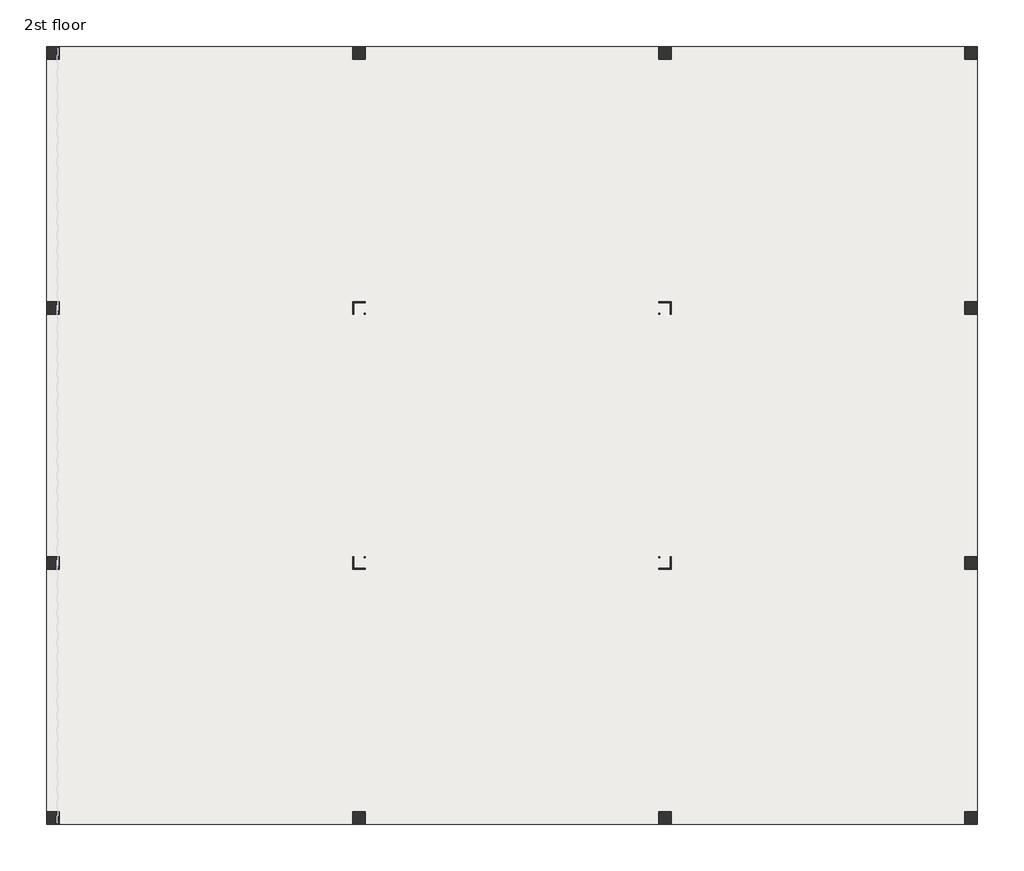
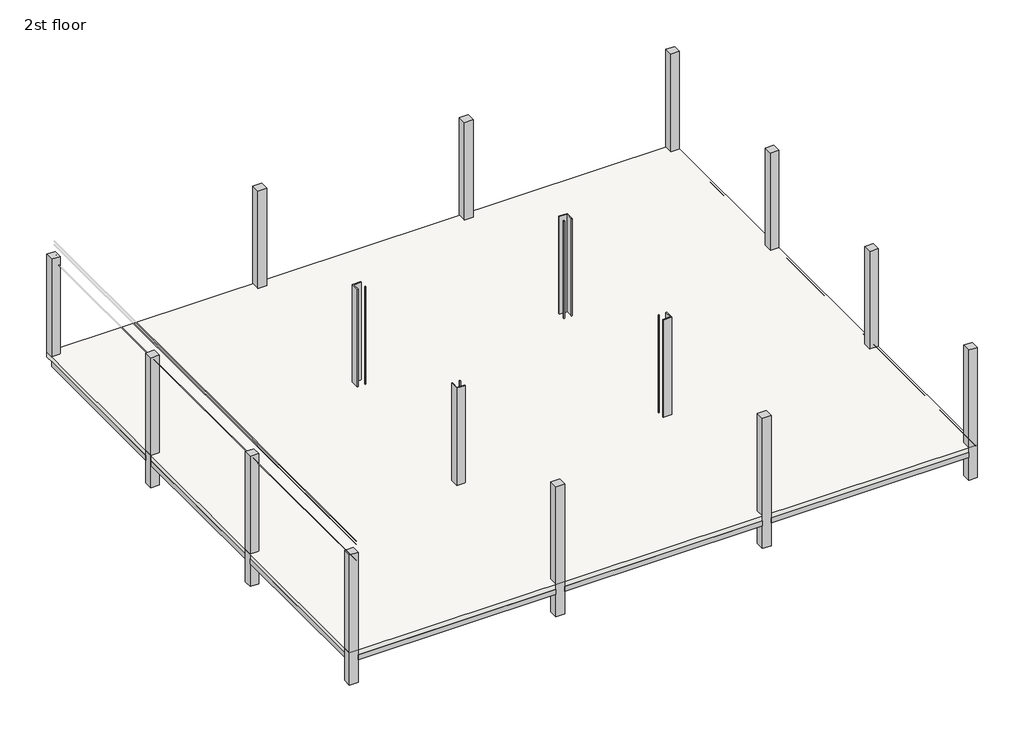
# One storey, part 1 of 2: 24 beams, 16 columns, 1 slab.
"""IFC4 building model written with IfcOpenShell, lengths in millimetres."""

from ifc_helpers import new_model, si_unit, frame, origin, place, context, project, spatial, polyline, outline, extrude, faceted_brep, element, save

model = new_model("IFC4")

# Units and contexts
model_context = context("Model", 3, world=origin())
ifc_project = project(units=[si_unit("LENGTHUNIT", "METRE", prefix="MILLI")], contexts=[model_context])

# Site, building, storey
site = spatial("IfcSite", under=ifc_project)
building = spatial("IfcBuilding", under=site)
storey = spatial("IfcBuildingStorey", under=building, Name="2st floor", Elevation=8500.0)

# Beams
placement = place(None, origin())
element("IfcBeam", 1, ObjectType="Concrete-Rectangular Beam : 250 x 300mm", at=placement, inside=storey, context=model_context, shape_type="SweptSolid", body=[
    extrude(outline(polyline([(-3083.7181639, -5443.2383613), (-3083.7181639, -5693.2383613), (-8833.7181639, -5693.2383613), (-8833.7181639, -5443.2383613), (-3083.7181639, -5443.2383613)])), frame((0.0, 0.0, 8200.0), z_axis=(0.0, 0.0, 1.0), x_axis=(1.0, 0.0, 0.0)), (0.0, 0.0, 1.0), 150.0),
])
element("IfcBeam", 2, ObjectType="Concrete-Rectangular Beam : 250 x 300mm", at=placement, inside=storey, context=model_context, shape_type="SweptSolid", body=[
    extrude(outline(polyline([(-2833.7181639, -5693.2383613), (-2833.7181639, -5443.2383613), (2916.2818361, -5443.2383613), (2916.2818361, -5693.2383613), (-2833.7181639, -5693.2383613)])), frame((0.0, 0.0, 8200.0), z_axis=(0.0, 0.0, 1.0), x_axis=(1.0, 0.0, 0.0)), (0.0, 0.0, 1.0), 150.0),
])
element("IfcBeam", 3, ObjectType="Concrete-Rectangular Beam : 250 x 300mm", at=placement, inside=storey, context=model_context, shape_type="SweptSolid", body=[
    extrude(outline(polyline([(3166.2818361, -5693.2383613), (3166.2818361, -5443.2383613), (8916.2818361, -5443.2383613), (8916.2818361, -5693.2383613), (3166.2818361, -5693.2383613)])), frame((0.0, 0.0, 8200.0), z_axis=(0.0, 0.0, 1.0), x_axis=(1.0, 0.0, 0.0)), (0.0, 0.0, 1.0), 150.0),
])
element("IfcBeam", 4, ObjectType="Concrete-Rectangular Beam : 250 x 300mm", at=placement, inside=storey, context=model_context, shape_type="SweptSolid", body=[
    extrude(outline(polyline([(-8833.7181639, -10443.2383613), (-9083.7181639, -10443.2383613), (-9083.7181639, -5693.2383613), (-8833.7181639, -5693.2383613), (-8833.7181639, -10443.2383613)])), frame((0.0, 0.0, 8200.0), z_axis=(0.0, 0.0, 1.0), x_axis=(1.0, 0.0, 0.0)), (0.0, 0.0, 1.0), 150.0),
])
element("IfcBeam", 5, ObjectType="Concrete-Rectangular Beam : 250 x 300mm", at=placement, inside=storey, context=model_context, shape_type="SweptSolid", body=[
    extrude(outline(polyline([(-8833.7181639, -15443.2383613), (-9083.7181639, -15443.2383613), (-9083.7181639, -10693.2383613), (-8833.7181639, -10693.2383613), (-8833.7181639, -15443.2383613)])), frame((0.0, 0.0, 8200.0), z_axis=(0.0, 0.0, 1.0), x_axis=(1.0, 0.0, 0.0)), (0.0, 0.0, 1.0), 150.0),
])
element("IfcBeam", 6, ObjectType="Concrete-Rectangular Beam : 250 x 300mm", at=placement, inside=storey, context=model_context, shape_type="SweptSolid", body=[
    extrude(outline(polyline([(-8833.7181639, -20443.2383613), (-9083.7181639, -20443.2383613), (-9083.7181639, -15693.2383613), (-8833.7181639, -15693.2383613), (-8833.7181639, -20443.2383613)])), frame((0.0, 0.0, 8200.0), z_axis=(0.0, 0.0, 1.0), x_axis=(1.0, 0.0, 0.0)), (0.0, 0.0, 1.0), 150.0),
])
element("IfcBeam", 7, ObjectType="Concrete-Rectangular Beam : 250 x 300mm", at=placement, inside=storey, context=model_context, shape_type="SweptSolid", body=[
    extrude(outline(polyline([(-2833.7181639, -10443.2383613), (-3083.7181639, -10443.2383613), (-3083.7181639, -5693.2383613), (-2833.7181639, -5693.2383613), (-2833.7181639, -10443.2383613)])), frame((0.0, 0.0, 8200.0), z_axis=(0.0, 0.0, 1.0), x_axis=(1.0, 0.0, 0.0)), (0.0, 0.0, 1.0), 150.0),
])
element("IfcBeam", 8, ObjectType="Concrete-Rectangular Beam : 250 x 300mm", at=placement, inside=storey, context=model_context, shape_type="SweptSolid", body=[
    extrude(outline(polyline([(-3083.7181639, -15443.2383613), (-3083.7181639, -10693.2383613), (-3058.7181639, -10693.2383613), (-3058.7181639, -15443.2383613), (-3083.7181639, -15443.2383613)])), frame((0.0, 0.0, 8200.0), z_axis=(0.0, 0.0, 1.0), x_axis=(1.0, 0.0, 0.0)), (0.0, 0.0, 1.0), 150.0),
    extrude(outline(polyline([(-2833.7181639, -10693.2383613), (-2833.7181639, -15443.2383613), (-2858.7181639, -15443.2383613), (-2858.7181639, -10693.2383613), (-2833.7181639, -10693.2383613)])), frame((0.0, 0.0, 8200.0), z_axis=(0.0, 0.0, 1.0), x_axis=(1.0, 0.0, 0.0)), (0.0, 0.0, 1.0), 150.0),
])
element("IfcBeam", 9, ObjectType="Concrete-Rectangular Beam : 250 x 300mm", at=placement, inside=storey, context=model_context, shape_type="SweptSolid", body=[
    extrude(outline(polyline([(-2833.7181639, -20443.2383613), (-3083.7181639, -20443.2383613), (-3083.7181639, -15693.2383613), (-2833.7181639, -15693.2383613), (-2833.7181639, -20443.2383613)])), frame((0.0, 0.0, 8200.0), z_axis=(0.0, 0.0, 1.0), x_axis=(1.0, 0.0, 0.0)), (0.0, 0.0, 1.0), 150.0),
])
element("IfcBeam", 10, ObjectType="Concrete-Rectangular Beam : 250 x 300mm", at=placement, inside=storey, context=model_context, shape_type="SweptSolid", body=[
    extrude(outline(polyline([(3166.2818361, -10443.2383613), (2916.2818361, -10443.2383613), (2916.2818361, -5693.2383613), (3166.2818361, -5693.2383613), (3166.2818361, -10443.2383613)])), frame((0.0, 0.0, 8200.0), z_axis=(0.0, 0.0, 1.0), x_axis=(1.0, 0.0, 0.0)), (0.0, 0.0, 1.0), 150.0),
])
element("IfcBeam", 11, ObjectType="Concrete-Rectangular Beam : 250 x 300mm", at=placement, inside=storey, context=model_context, shape_type="SweptSolid", body=[
    extrude(outline(polyline([(2916.2818361, -15443.2383613), (2916.2818361, -10693.2383613), (2941.2818361, -10693.2383613), (2941.2818361, -15443.2383613), (2916.2818361, -15443.2383613)])), frame((0.0, 0.0, 8200.0), z_axis=(0.0, 0.0, 1.0), x_axis=(1.0, 0.0, 0.0)), (0.0, 0.0, 1.0), 150.0),
    extrude(outline(polyline([(3166.2818361, -10693.2383613), (3166.2818361, -15443.2383613), (3141.2818361, -15443.2383613), (3141.2818361, -10693.2383613), (3166.2818361, -10693.2383613)])), frame((0.0, 0.0, 8200.0), z_axis=(0.0, 0.0, 1.0), x_axis=(1.0, 0.0, 0.0)), (0.0, 0.0, 1.0), 150.0),
])
element("IfcBeam", 12, ObjectType="Concrete-Rectangular Beam : 250 x 300mm", at=placement, inside=storey, context=model_context, shape_type="SweptSolid", body=[
    extrude(outline(polyline([(3166.2818361, -20443.2383613), (2916.2818361, -20443.2383613), (2916.2818361, -15693.2383613), (3166.2818361, -15693.2383613), (3166.2818361, -20443.2383613)])), frame((0.0, 0.0, 8200.0), z_axis=(0.0, 0.0, 1.0), x_axis=(1.0, 0.0, 0.0)), (0.0, 0.0, 1.0), 150.0),
])
element("IfcBeam", 13, ObjectType="Concrete-Rectangular Beam : 250 x 300mm", at=placement, inside=storey, context=model_context, shape_type="SweptSolid", body=[
    extrude(outline(polyline([(9166.2818361, -10443.2383613), (8916.2818361, -10443.2383613), (8916.2818361, -5693.2383613), (9166.2818361, -5693.2383613), (9166.2818361, -10443.2383613)])), frame((0.0, 0.0, 8200.0), z_axis=(0.0, 0.0, 1.0), x_axis=(1.0, 0.0, 0.0)), (0.0, 0.0, 1.0), 150.0),
])
element("IfcBeam", 14, ObjectType="Concrete-Rectangular Beam : 250 x 300mm", at=placement, inside=storey, context=model_context, shape_type="SweptSolid", body=[
    extrude(outline(polyline([(9166.2818361, -15443.2383613), (8916.2818361, -15443.2383613), (8916.2818361, -10693.2383613), (9166.2818361, -10693.2383613), (9166.2818361, -15443.2383613)])), frame((0.0, 0.0, 8200.0), z_axis=(0.0, 0.0, 1.0), x_axis=(1.0, 0.0, 0.0)), (0.0, 0.0, 1.0), 150.0),
])
element("IfcBeam", 15, ObjectType="Concrete-Rectangular Beam : 250 x 300mm", at=placement, inside=storey, context=model_context, shape_type="SweptSolid", body=[
    extrude(outline(polyline([(9166.2818361, -20443.2383613), (8916.2818361, -20443.2383613), (8916.2818361, -15693.2383613), (9166.2818361, -15693.2383613), (9166.2818361, -20443.2383613)])), frame((0.0, 0.0, 8200.0), z_axis=(0.0, 0.0, 1.0), x_axis=(1.0, 0.0, 0.0)), (0.0, 0.0, 1.0), 150.0),
])
element("IfcBeam", 16, ObjectType="Concrete-Rectangular Beam : 250 x 300mm", at=placement, inside=storey, context=model_context, shape_type="SweptSolid", body=[
    extrude(outline(polyline([(-8833.7181639, -20693.2383613), (-8833.7181639, -20443.2383613), (-3083.7181639, -20443.2383613), (-3083.7181639, -20693.2383613), (-8833.7181639, -20693.2383613)])), frame((0.0, 0.0, 8200.0), z_axis=(0.0, 0.0, 1.0), x_axis=(1.0, 0.0, 0.0)), (0.0, 0.0, 1.0), 150.0),
])
element("IfcBeam", 17, ObjectType="Concrete-Rectangular Beam : 250 x 300mm", at=placement, inside=storey, context=model_context, shape_type="SweptSolid", body=[
    extrude(outline(polyline([(-2833.7181639, -20693.2383613), (-2833.7181639, -20443.2383613), (2916.2818361, -20443.2383613), (2916.2818361, -20693.2383613), (-2833.7181639, -20693.2383613)])), frame((0.0, 0.0, 8200.0), z_axis=(0.0, 0.0, 1.0), x_axis=(1.0, 0.0, 0.0)), (0.0, 0.0, 1.0), 150.0),
])
element("IfcBeam", 18, ObjectType="Concrete-Rectangular Beam : 250 x 300mm", at=placement, inside=storey, context=model_context, shape_type="SweptSolid", body=[
    extrude(outline(polyline([(3166.2818361, -20693.2383613), (3166.2818361, -20443.2383613), (8916.2818361, -20443.2383613), (8916.2818361, -20693.2383613), (3166.2818361, -20693.2383613)])), frame((0.0, 0.0, 8200.0), z_axis=(0.0, 0.0, 1.0), x_axis=(1.0, 0.0, 0.0)), (0.0, 0.0, 1.0), 150.0),
])
element("IfcBeam", 19, ObjectType="Concrete-Rectangular Beam : 250 x 300mm", at=placement, inside=storey, context=model_context, shape_type="SweptSolid", body=[
    extrude(outline(polyline([(-8833.7181639, -15693.2383613), (-8833.7181639, -15443.2383613), (-3083.7181639, -15443.2383613), (-3083.7181639, -15693.2383613), (-8833.7181639, -15693.2383613)])), frame((0.0, 0.0, 8200.0), z_axis=(0.0, 0.0, 1.0), x_axis=(1.0, 0.0, 0.0)), (0.0, 0.0, 1.0), 150.0),
])
element("IfcBeam", 20, ObjectType="Concrete-Rectangular Beam : 250 x 300mm", at=placement, inside=storey, context=model_context, shape_type="SweptSolid", body=[
    extrude(outline(polyline([(2916.2818361, -15693.2383613), (-2833.7181639, -15693.2383613), (-2833.7181639, -15668.2383613), (2916.2818361, -15668.2383613), (2916.2818361, -15693.2383613)])), frame((0.0, 0.0, 8200.0), z_axis=(0.0, 0.0, 1.0), x_axis=(1.0, 0.0, 0.0)), (0.0, 0.0, 1.0), 150.0),
    extrude(outline(polyline([(-2833.7181639, -15443.2383613), (2916.2818361, -15443.2383613), (2916.2818361, -15468.2383613), (-2833.7181639, -15468.2383613), (-2833.7181639, -15443.2383613)])), frame((0.0, 0.0, 8200.0), z_axis=(0.0, 0.0, 1.0), x_axis=(1.0, 0.0, 0.0)), (0.0, 0.0, 1.0), 150.0),
])
element("IfcBeam", 21, ObjectType="Concrete-Rectangular Beam : 250 x 300mm", at=placement, inside=storey, context=model_context, shape_type="SweptSolid", body=[
    extrude(outline(polyline([(3166.2818361, -15693.2383613), (3166.2818361, -15443.2383613), (8916.2818361, -15443.2383613), (8916.2818361, -15693.2383613), (3166.2818361, -15693.2383613)])), frame((0.0, 0.0, 8200.0), z_axis=(0.0, 0.0, 1.0), x_axis=(1.0, 0.0, 0.0)), (0.0, 0.0, 1.0), 150.0),
])
element("IfcBeam", 22, ObjectType="Concrete-Rectangular Beam : 250 x 300mm", at=placement, inside=storey, context=model_context, shape_type="SweptSolid", body=[
    extrude(outline(polyline([(-8833.7181639, -10693.2383613), (-8833.7181639, -10443.2383613), (-3083.7181639, -10443.2383613), (-3083.7181639, -10693.2383613), (-8833.7181639, -10693.2383613)])), frame((0.0, 0.0, 8200.0), z_axis=(0.0, 0.0, 1.0), x_axis=(1.0, 0.0, 0.0)), (0.0, 0.0, 1.0), 150.0),
])
element("IfcBeam", 23, ObjectType="Concrete-Rectangular Beam : 250 x 300mm", at=placement, inside=storey, context=model_context, shape_type="SweptSolid", body=[
    extrude(outline(polyline([(2916.2818361, -10693.2383613), (-2833.7181639, -10693.2383613), (-2833.7181639, -10668.2383613), (2916.2818361, -10668.2383613), (2916.2818361, -10693.2383613)])), frame((0.0, 0.0, 8200.0), z_axis=(0.0, 0.0, 1.0), x_axis=(1.0, 0.0, 0.0)), (0.0, 0.0, 1.0), 150.0),
    extrude(outline(polyline([(-2833.7181639, -10443.2383613), (2916.2818361, -10443.2383613), (2916.2818361, -10468.2383613), (-2833.7181639, -10468.2383613), (-2833.7181639, -10443.2383613)])), frame((0.0, 0.0, 8200.0), z_axis=(0.0, 0.0, 1.0), x_axis=(1.0, 0.0, 0.0)), (0.0, 0.0, 1.0), 150.0),
])
element("IfcBeam", 24, ObjectType="Concrete-Rectangular Beam : 250 x 300mm", at=placement, inside=storey, context=model_context, shape_type="SweptSolid", body=[
    extrude(outline(polyline([(3166.2818361, -10693.2383613), (3166.2818361, -10443.2383613), (8916.2818361, -10443.2383613), (8916.2818361, -10693.2383613), (3166.2818361, -10693.2383613)])), frame((0.0, 0.0, 8200.0), z_axis=(0.0, 0.0, 1.0), x_axis=(1.0, 0.0, 0.0)), (0.0, 0.0, 1.0), 150.0),
])

# Columns
element("IfcColumn", 25, ObjectType="Concrete-Rectangular-Column : 250x250 mm", at=placement, inside=storey, context=model_context, shape_type="SweptSolid", body=[
    extrude(outline(polyline([(-8833.7181639, -20443.2383613), (-8833.7181639, -20693.2383613), (-9083.7181639, -20693.2383613), (-9083.7181639, -20443.2383613), (-8833.7181639, -20443.2383613)])), frame((0.0, 0.0, 7500.0), z_axis=(0.0, 0.0, 1.0), x_axis=(1.0, 0.0, 0.0)), (0.0, 0.0, 1.0), 4000.0),
])
element("IfcColumn", 26, ObjectType="Concrete-Rectangular-Column : 250x250 mm", at=placement, inside=storey, context=model_context, shape_type="SweptSolid", body=[
    extrude(outline(polyline([(-8833.7181639, -15443.2383613), (-8833.7181639, -15693.2383613), (-9083.7181639, -15693.2383613), (-9083.7181639, -15443.2383613), (-8833.7181639, -15443.2383613)])), frame((0.0, 0.0, 7500.0), z_axis=(0.0, 0.0, 1.0), x_axis=(1.0, 0.0, 0.0)), (0.0, 0.0, 1.0), 4000.0),
])
element("IfcColumn", 27, ObjectType="Concrete-Rectangular-Column : 250x250 mm", at=placement, inside=storey, context=model_context, shape_type="SweptSolid", body=[
    extrude(outline(polyline([(-8833.7181639, -10443.2383613), (-8833.7181639, -10693.2383613), (-9083.7181639, -10693.2383613), (-9083.7181639, -10443.2383613), (-8833.7181639, -10443.2383613)])), frame((0.0, 0.0, 7500.0), z_axis=(0.0, 0.0, 1.0), x_axis=(1.0, 0.0, 0.0)), (0.0, 0.0, 1.0), 4000.0),
])
element("IfcColumn", 28, ObjectType="Concrete-Rectangular-Column : 250x250 mm", at=placement, inside=storey, context=model_context, shape_type="SweptSolid", body=[
    extrude(outline(polyline([(-8833.7181639, -5443.2383613), (-8833.7181639, -5693.2383613), (-9083.7181639, -5693.2383613), (-9083.7181639, -5443.2383613), (-8833.7181639, -5443.2383613)])), frame((0.0, 0.0, 8500.0), z_axis=(0.0, 0.0, 1.0), x_axis=(1.0, 0.0, 0.0)), (0.0, 0.0, 1.0), 3000.0),
])
element("IfcColumn", 29, ObjectType="Concrete-Rectangular-Column : 250x250 mm", at=placement, inside=storey, context=model_context, shape_type="SweptSolid", body=[
    extrude(outline(polyline([(-2833.7181639, -20443.2383613), (-2833.7181639, -20693.2383613), (-3083.7181639, -20693.2383613), (-3083.7181639, -20443.2383613), (-2833.7181639, -20443.2383613)])), frame((0.0, 0.0, 7500.0), z_axis=(0.0, 0.0, 1.0), x_axis=(1.0, 0.0, 0.0)), (0.0, 0.0, 1.0), 4000.0),
])
element("IfcColumn", 30, ObjectType="Concrete-Rectangular-Column : 250x250 mm", at=placement, inside=storey, context=model_context, shape_type="SweptSolid", body=[
    extrude(outline(polyline([(-2833.7181639, -15443.2383613), (-2833.7181639, -15468.2383613), (-2858.7181639, -15468.2383613), (-2858.7181639, -15443.2383613), (-2833.7181639, -15443.2383613)])), frame((0.0, 0.0, 7500.0), z_axis=(0.0, 0.0, 1.0), x_axis=(1.0, 0.0, 0.0)), (0.0, 0.0, 1.0), 4000.0),
    extrude(outline(polyline([(-2833.7181639, -15693.2383613), (-3083.7181639, -15693.2383613), (-3083.7181639, -15443.2383613), (-3058.7181639, -15443.2383613), (-3058.7181639, -15668.2383613), (-2833.7181639, -15668.2383613), (-2833.7181639, -15693.2383613)])), frame((0.0, 0.0, 7500.0), z_axis=(0.0, 0.0, 1.0), x_axis=(1.0, 0.0, 0.0)), (0.0, 0.0, 1.0), 4000.0),
])
element("IfcColumn", 31, ObjectType="Concrete-Rectangular-Column : 250x250 mm", at=placement, inside=storey, context=model_context, shape_type="SweptSolid", body=[
    extrude(outline(polyline([(-3083.7181639, -10693.2383613), (-3083.7181639, -10443.2383613), (-2833.7181639, -10443.2383613), (-2833.7181639, -10468.2383613), (-3058.7181639, -10468.2383613), (-3058.7181639, -10693.2383613), (-3083.7181639, -10693.2383613)])), frame((0.0, 0.0, 7500.0), z_axis=(0.0, 0.0, 1.0), x_axis=(1.0, 0.0, 0.0)), (0.0, 0.0, 1.0), 4000.0),
    extrude(outline(polyline([(-2833.7181639, -10668.2383613), (-2833.7181639, -10693.2383613), (-2858.7181639, -10693.2383613), (-2858.7181639, -10668.2383613), (-2833.7181639, -10668.2383613)])), frame((0.0, 0.0, 7500.0), z_axis=(0.0, 0.0, 1.0), x_axis=(1.0, 0.0, 0.0)), (0.0, 0.0, 1.0), 4000.0),
])
element("IfcColumn", 32, ObjectType="Concrete-Rectangular-Column : 250x250 mm", at=placement, inside=storey, context=model_context, shape_type="SweptSolid", body=[
    extrude(outline(polyline([(-2833.7181639, -5443.2383613), (-2833.7181639, -5693.2383613), (-3083.7181639, -5693.2383613), (-3083.7181639, -5443.2383613), (-2833.7181639, -5443.2383613)])), frame((0.0, 0.0, 7500.0), z_axis=(0.0, 0.0, 1.0), x_axis=(1.0, 0.0, 0.0)), (0.0, 0.0, 1.0), 4000.0),
])
element("IfcColumn", 33, ObjectType="Concrete-Rectangular-Column : 250x250 mm", at=placement, inside=storey, context=model_context, shape_type="SweptSolid", body=[
    extrude(outline(polyline([(3166.2818361, -20443.2383613), (3166.2818361, -20693.2383613), (2916.2818361, -20693.2383613), (2916.2818361, -20443.2383613), (3166.2818361, -20443.2383613)])), frame((0.0, 0.0, 7500.0), z_axis=(0.0, 0.0, 1.0), x_axis=(1.0, 0.0, 0.0)), (0.0, 0.0, 1.0), 4000.0),
])
element("IfcColumn", 34, ObjectType="Concrete-Rectangular-Column : 250x250 mm", at=placement, inside=storey, context=model_context, shape_type="SweptSolid", body=[
    extrude(outline(polyline([(2916.2818361, -15468.2383613), (2916.2818361, -15443.2383613), (2941.2818361, -15443.2383613), (2941.2818361, -15468.2383613), (2916.2818361, -15468.2383613)])), frame((0.0, 0.0, 7500.0), z_axis=(0.0, 0.0, 1.0), x_axis=(1.0, 0.0, 0.0)), (0.0, 0.0, 1.0), 4000.0),
    extrude(outline(polyline([(3166.2818361, -15443.2383613), (3166.2818361, -15693.2383613), (2916.2818361, -15693.2383613), (2916.2818361, -15668.2383613), (3141.2818361, -15668.2383613), (3141.2818361, -15443.2383613), (3166.2818361, -15443.2383613)])), frame((0.0, 0.0, 7500.0), z_axis=(0.0, 0.0, 1.0), x_axis=(1.0, 0.0, 0.0)), (0.0, 0.0, 1.0), 4000.0),
])
element("IfcColumn", 35, ObjectType="Concrete-Rectangular-Column : 250x250 mm", at=placement, inside=storey, context=model_context, shape_type="SweptSolid", body=[
    extrude(outline(polyline([(3166.2818361, -10443.2383613), (3166.2818361, -10693.2383613), (3141.2818361, -10693.2383613), (3141.2818361, -10468.2383613), (2916.2818361, -10468.2383613), (2916.2818361, -10443.2383613), (3166.2818361, -10443.2383613)])), frame((0.0, 0.0, 7500.0), z_axis=(0.0, 0.0, 1.0), x_axis=(1.0, 0.0, 0.0)), (0.0, 0.0, 1.0), 4000.0),
    extrude(outline(polyline([(2916.2818361, -10693.2383613), (2916.2818361, -10668.2383613), (2941.2818361, -10668.2383613), (2941.2818361, -10693.2383613), (2916.2818361, -10693.2383613)])), frame((0.0, 0.0, 7500.0), z_axis=(0.0, 0.0, 1.0), x_axis=(1.0, 0.0, 0.0)), (0.0, 0.0, 1.0), 4000.0),
])
element("IfcColumn", 36, ObjectType="Concrete-Rectangular-Column : 250x250 mm", at=placement, inside=storey, context=model_context, shape_type="SweptSolid", body=[
    extrude(outline(polyline([(3166.2818361, -5443.2383613), (3166.2818361, -5693.2383613), (2916.2818361, -5693.2383613), (2916.2818361, -5443.2383613), (3166.2818361, -5443.2383613)])), frame((0.0, 0.0, 7500.0), z_axis=(0.0, 0.0, 1.0), x_axis=(1.0, 0.0, 0.0)), (0.0, 0.0, 1.0), 4000.0),
])
element("IfcColumn", 37, ObjectType="Concrete-Rectangular-Column : 250x250 mm", at=placement, inside=storey, context=model_context, shape_type="SweptSolid", body=[
    extrude(outline(polyline([(9166.2818361, -20443.2383613), (9166.2818361, -20693.2383613), (8916.2818361, -20693.2383613), (8916.2818361, -20443.2383613), (9166.2818361, -20443.2383613)])), frame((0.0, 0.0, 7500.0), z_axis=(0.0, 0.0, 1.0), x_axis=(1.0, 0.0, 0.0)), (0.0, 0.0, 1.0), 4000.0),
])
element("IfcColumn", 38, ObjectType="Concrete-Rectangular-Column : 250x250 mm", at=placement, inside=storey, context=model_context, shape_type="SweptSolid", body=[
    extrude(outline(polyline([(9166.2818361, -15443.2383613), (9166.2818361, -15693.2383613), (8916.2818361, -15693.2383613), (8916.2818361, -15443.2383613), (9166.2818361, -15443.2383613)])), frame((0.0, 0.0, 7500.0), z_axis=(0.0, 0.0, 1.0), x_axis=(1.0, 0.0, 0.0)), (0.0, 0.0, 1.0), 4000.0),
])
element("IfcColumn", 39, ObjectType="Concrete-Rectangular-Column : 250x250 mm", at=placement, inside=storey, context=model_context, shape_type="SweptSolid", body=[
    extrude(outline(polyline([(9166.2818361, -10443.2383613), (9166.2818361, -10693.2383613), (8916.2818361, -10693.2383613), (8916.2818361, -10443.2383613), (9166.2818361, -10443.2383613)])), frame((0.0, 0.0, 7500.0), z_axis=(0.0, 0.0, 1.0), x_axis=(1.0, 0.0, 0.0)), (0.0, 0.0, 1.0), 4000.0),
])
element("IfcColumn", 40, ObjectType="Concrete-Rectangular-Column : 250x250 mm", at=placement, inside=storey, context=model_context, shape_type="SweptSolid", body=[
    extrude(outline(polyline([(9166.2818361, -5443.2383613), (9166.2818361, -5693.2383613), (8916.2818361, -5693.2383613), (8916.2818361, -5443.2383613), (9166.2818361, -5443.2383613)])), frame((0.0, 0.0, 7500.0), z_axis=(0.0, 0.0, 1.0), x_axis=(1.0, 0.0, 0.0)), (0.0, 0.0, 1.0), 4000.0),
])

# Slab
element("IfcSlab", 41, ObjectType="150mm Foundation Slab", at=placement, inside=storey, context=model_context, shape_type="Brep", body=[
    faceted_brep([(-9083.7181639, -5443.2383613, 8350.0), (-8833.7181639, -5443.2383613, 8350.0), (-3083.7181639, -5443.2383613, 8350.0), (-2833.7181639, -5443.2383613, 8350.0), (2916.2818361, -5443.2383613, 8350.0), (3166.2818361, -5443.2383613, 8350.0), (8916.2818361, -5443.2383613, 8350.0), (9166.2818361, -5443.2383613, 8350.0), (9166.2818361, -5693.2383613, 8350.0), (9166.2818361, -10443.2383613, 8350.0), (9166.2818361, -10693.2383613, 8350.0), (9166.2818361, -15443.2383613, 8350.0), (9166.2818361, -15693.2383613, 8350.0), (9166.2818361, -20443.2383613, 8350.0), (9166.2818361, -20693.2383613, 8350.0), (8916.2818361, -20693.2383613, 8350.0), (3166.2818361, -20693.2383613, 8350.0), (2916.2818361, -20693.2383613, 8350.0), (-2833.7181639, -20693.2383613, 8350.0), (-3083.7181639, -20693.2383613, 8350.0), (-8833.7181639, -20693.2383613, 8350.0), (-9083.7181639, -20693.2383613, 8350.0), (-9083.7181639, -20443.2383613, 8350.0), (-9083.7181639, -15693.2383613, 8350.0), (-9083.7181639, -15443.2383613, 8350.0), (-9083.7181639, -10693.2383613, 8350.0), (-9083.7181639, -10443.2383613, 8350.0), (-9083.7181639, -5693.2383613, 8350.0), (-9083.7181639, -5443.2383613, 8500.0), (-9083.7181639, -20693.2383613, 8500.0), (9166.2818361, -20693.2383613, 8500.0), (9166.2818361, -5443.2383613, 8500.0)], [[[0, 1, 2, 3, 4, 5, 6, 7, 8, 9, 10, 11, 12, 13, 14, 15, 16, 17, 18, 19, 20, 21, 22, 23, 24, 25, 26, 27]], [[28, 29, 30, 31]], [[7, 6, 5, 4, 3, 2, 1, 0, 28, 31]], [[14, 13, 12, 11, 10, 9, 8, 7, 31, 30]], [[21, 20, 19, 18, 17, 16, 15, 14, 30, 29]], [[0, 27, 26, 25, 24, 23, 22, 21, 29, 28]]]),
])

save(model, "model.ifc")

# Revit data of these elements
# Type "Concrete-Rectangular Beam : 250 x 300mm"
#   Length [instance default] = 1524 mm
#   b = 250 mm
#   h = 300 mm
#   Structural Material [instance default] = Concrete, Cast-in-Place gray
#   Assembly Code = ""
# Type "Concrete-Rectangular-Column : 250x250 mm"
#   b = 250 mm
#   h = 250 mm
#   Structural Material [instance default] = Concrete, Cast-in-Place gray
# Type "150mm Foundation Slab"
#   Layers, outside or top first: 150 mm "Concrete, Cast-in-Place gray" (function 1)
# Elements 1, 2, 3, 4, 5, 6, 7, 8, 9, 10, 11, 12, 13, 14, 15, 16, 17, 18, 19, 20, 21, 22, 23, 24 (IfcBeam, "Concrete-Rectangular Beam : 250 x 300mm")
#   Structural Material = Concrete, Cast-in-Place gray
#   Phase Created = New Construction
#   Materials on its faces: "Concrete, Cast-in-Place gray"
# Elements 25, 26, 27, 28, 29, 30, 31, 32, 33, 34, 35, 36, 37, 38, 39, 40 (IfcColumn, "Concrete-Rectangular-Column : 250x250 mm")
#   Structural Material = Concrete, Cast-in-Place gray
#   Phase Created = New Construction
#   Materials on its faces: "Concrete, Cast-in-Place gray"
# Element 41 (IfcSlab, "150mm Foundation Slab")
#   built-in parameter 1001955 = 3.14159 (stored number, unit not read)
#   Height Offset From Level = 0 mm
#   built-in parameter 1001954 = 1
#   Phase Created = New Construction
#   Materials on its faces: "Concrete, Cast-in-Place gray"
# Materials
#   "Concrete, Cast-in-Place gray": class "Concrete", colour RGB 192 192 192, transparency 0, Description = "Cast-in-place concrete", Cost = 0
